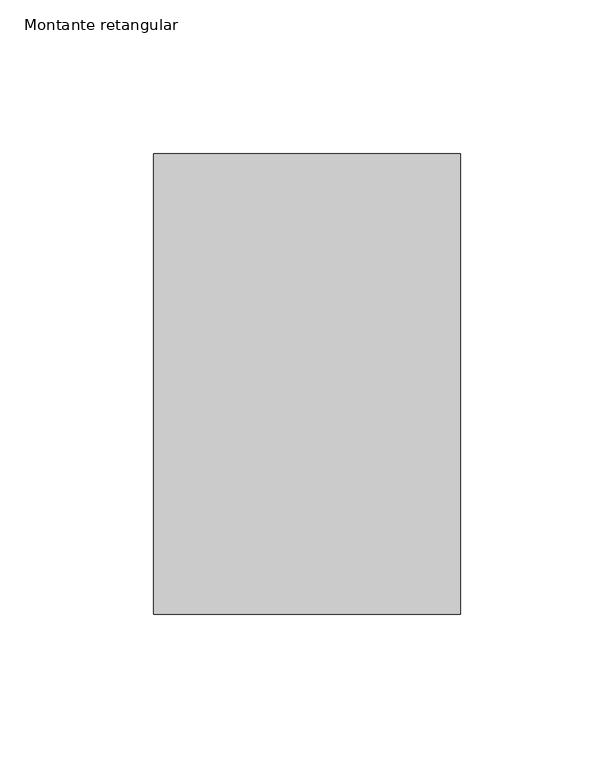
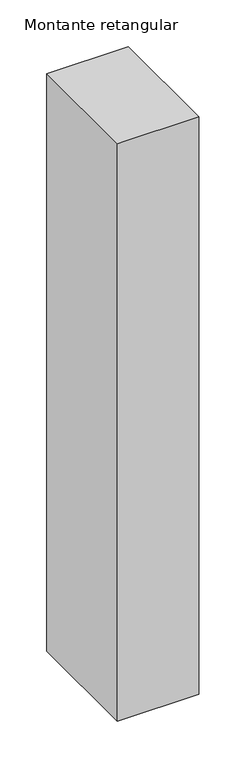
"""IFC4 building model written with IfcOpenShell, lengths in millimetres: member geometry, Montante retangular : CC_100 X 150  mm."""

import ifcopenshell
import ifcopenshell.guid

model = None  # the IFC model being written
_history = None  # IfcOwnerHistory: only IFC2X3 demands one
_inside = {}  # id of a spatial element -> (the spatial element, [elements in it])
_under = {}  # id of a project, library or spatial element -> (it, [spatial elements below it])
_declared = {}  # id of a project -> (the project, [libraries it declares])
_typed = {}  # id of a type object -> (the type object, [elements of that type])
_made_of = {}  # id of a material, layer set ... -> (it, [elements and type objects made of it])


def new_model(schema):
    """Start an empty IFC model of exactly this schema.

    Asked for "IFC4X3", IfcOpenShell would pick the latest addendum, in which some entities
    have other attributes; the version numbers below select the first issue.
    IFC2X3 requires an IfcOwnerHistory on every rooted entity: one is made here for all.
    """
    global model, _history
    if schema == "IFC4X3":
        model = ifcopenshell.file(schema_version=(4, 3, 0, 0))
    else:
        model = ifcopenshell.file(schema=schema)
    _inside.clear()
    _under.clear()
    _declared.clear()
    _typed.clear()
    _made_of.clear()
    _history = None
    if model.schema == "IFC2X3":
        org = make("IfcOrganization", Name="unknown")
        user = make(
            "IfcPersonAndOrganization",
            ThePerson=make("IfcPerson", FamilyName="unknown"),
            TheOrganization=org,
        )
        app = make(
            "IfcApplication",
            ApplicationDeveloper=org,
            Version="unknown",
            ApplicationFullName="unknown",
            ApplicationIdentifier="unknown",
        )
        _history = make(
            "IfcOwnerHistory",
            OwningUser=user,
            OwningApplication=app,
            ChangeAction="ADDED",
            CreationDate=0,
        )
    return model


def make(cls, **values):
    """One entity of the class cls with the attributes given. An attribute that is None is left unset."""
    return model.create_entity(
        cls, **{name: value for name, value in values.items() if value is not None}
    )


def rooted(cls, **values):
    """An entity with a GlobalId (a new one), such as an element, a storey or a relation."""
    return make(cls, GlobalId=ifcopenshell.guid.new(), OwnerHistory=_history, **values)


def si_unit(unit_type, name, prefix=None):
    """IfcSIUnit, for example si_unit("LENGTHUNIT", "METRE", prefix="MILLI")."""
    return make("IfcSIUnit", UnitType=unit_type, Prefix=prefix, Name=name)


def assignment(units):
    """IfcUnitAssignment: the units of a project."""
    return None if units is None else make("IfcUnitAssignment", Units=units)


def point(xyz):
    """IfcCartesianPoint."""
    return None if xyz is None else make("IfcCartesianPoint", Coordinates=xyz)


def direction(xyz):
    """IfcDirection."""
    return None if xyz is None else make("IfcDirection", DirectionRatios=xyz)


def frame(location, z_axis=None, x_axis=None):
    """IfcAxis2Placement3D, a coordinate frame: its origin and axes. An axis left out is left unset."""
    return make(
        "IfcAxis2Placement3D",
        Location=point(location),
        Axis=direction(z_axis),
        RefDirection=direction(x_axis),
    )


def origin():
    """The frame at (0, 0, 0) with its axes left unset."""
    return frame((0.0, 0.0, 0.0))


def place(relative_to, where):
    """IfcLocalPlacement: puts the frame where relative to a parent placement (None: the world)."""
    return make(
        "IfcLocalPlacement", PlacementRelTo=relative_to, RelativePlacement=where
    )


def context(
    kind, dimensions, precision=None, world=None, true_north=None, identifier=None
):
    """IfcGeometricRepresentationContext, for example the 3D "Model" context."""
    return make(
        "IfcGeometricRepresentationContext",
        ContextIdentifier=identifier,
        ContextType=kind,
        CoordinateSpaceDimension=dimensions,
        Precision=precision,
        WorldCoordinateSystem=world,
        TrueNorth=true_north,
    )


def project(units=None, contexts=None):
    """IfcProject with its units and contexts."""
    return rooted(
        "IfcProject",
        Name="project",
        RepresentationContexts=contexts,
        UnitsInContext=assignment(units),
    )


def spatial(cls, under=None, at=None, **own):
    """A site, building, storey or space (cls), placed at a placement, below another one or the project."""
    s = rooted(cls, ObjectPlacement=at, **own)
    if under is not None:
        _under.setdefault(under.id(), (under, []))[1].append(s)
    return s


def polyline(points):
    """IfcPolyline through the points."""
    return make("IfcPolyline", Points=[point(p) for p in points])


def outline(outer, holes=None, kind="AREA"):
    """IfcArbitraryClosedProfileDef: a profile drawn as a closed curve; with holes, ...WithVoids."""
    if holes is None:
        return make("IfcArbitraryClosedProfileDef", ProfileType=kind, OuterCurve=outer)
    return make(
        "IfcArbitraryProfileDefWithVoids",
        ProfileType=kind,
        OuterCurve=outer,
        InnerCurves=holes,
    )


def extrude(swept, where, along, depth):
    """IfcExtrudedAreaSolid: the profile swept, set in the frame where, extruded along a direction by depth."""
    return make(
        "IfcExtrudedAreaSolid",
        SweptArea=swept,
        Position=where,
        ExtrudedDirection=direction(along),
        Depth=depth,
    )


def shape(context_of_items, identifier, shape_type, items):
    """IfcShapeRepresentation: the items that make up one representation, for example the "Body"."""
    return make(
        "IfcShapeRepresentation",
        ContextOfItems=context_of_items,
        RepresentationIdentifier=identifier,
        RepresentationType=shape_type,
        Items=items,
    )


def source(mapping_origin, context_of_items, identifier, shape_type, items):
    """IfcRepresentationMap: a shape defined once, which mapped items show again and again."""
    return make(
        "IfcRepresentationMap",
        MappingOrigin=mapping_origin,
        MappedRepresentation=shape(context_of_items, identifier, shape_type, items),
    )


def transform(
    local_origin,
    x_axis=None,
    y_axis=None,
    z_axis=None,
    scale=None,
    scale2=None,
    scale3=None,
    uniform=True,
):
    """IfcCartesianTransformationOperator3D, or its non-uniform kind. x_axis, y_axis, z_axis: its Axis1, 2, 3."""
    if uniform:
        return make(
            "IfcCartesianTransformationOperator3D",
            Axis1=direction(x_axis),
            Axis2=direction(y_axis),
            LocalOrigin=point(local_origin),
            Scale=scale,
            Axis3=direction(z_axis),
        )
    return make(
        "IfcCartesianTransformationOperator3DnonUniform",
        Axis1=direction(x_axis),
        Axis2=direction(y_axis),
        LocalOrigin=point(local_origin),
        Scale=scale,
        Axis3=direction(z_axis),
        Scale2=scale2,
        Scale3=scale3,
    )


def mapped(mapping_source, mapping_target):
    """IfcMappedItem: shows the shape of a source again, moved by a transform."""
    return make(
        "IfcMappedItem", MappingSource=mapping_source, MappingTarget=mapping_target
    )


def made_of(thing, what):
    """Note that an element or type object is made of a material, layer set ...; save() writes the relation."""
    if what is not None:
        _made_of.setdefault(what.id(), (what, []))[1].append(thing)
    return thing


def element(
    cls,
    number,
    at=None,
    inside=None,
    cuts=None,
    type_object=None,
    material=None,
    context=None,
    identifier="Body",
    shape_type=None,
    held_by="IfcProductDefinitionShape",
    body=None,
    shapes=None,
    **own,
):
    """One element of the class cls, such as IfcWall. Its Tag is "e" and its number.

    at: its placement. inside: the storey or other place that contains it. cuts: it is an
    opening in that element (IfcRelVoidsElement). A single representation is given by context,
    identifier, shape_type and body (its items); several are given by shapes. held_by: the class
    of the entity that holds the representations. save() writes the other relations.
    """
    e = rooted(cls, Tag="e%d" % number, ObjectPlacement=at, **own)
    if body is not None:
        shapes = [shape(context, identifier, shape_type, body)]
    if shapes is not None:
        e.Representation = make(held_by, Representations=shapes)
    if inside is not None:
        _inside.setdefault(inside.id(), (inside, []))[1].append(e)
    if cuts is not None:
        rooted(
            "IfcRelVoidsElement", RelatingBuildingElement=cuts, RelatedOpeningElement=e
        )
    if type_object is not None:
        _typed.setdefault(type_object.id(), (type_object, []))[1].append(e)
    return made_of(e, material)


def aggregate(whole, parts):
    """IfcRelAggregates: a whole, such as a stair, and the parts it consists of."""
    return rooted("IfcRelAggregates", RelatingObject=whole, RelatedObjects=parts)


def save(model, path):
    """Write the relations noted so far, then the file.

    IfcRelAggregates (storeys below a building ...), IfcRelContainedInSpatialStructure (elements
    in a storey), IfcRelDefinesByType, IfcRelAssociatesMaterial and IfcRelDeclares: one each for
    every whole, place, type object, material and project.
    """
    for whole, parts in _under.values():
        aggregate(whole, parts)
    for where, things in _inside.values():
        rooted(
            "IfcRelContainedInSpatialStructure",
            RelatedElements=things,
            RelatingStructure=where,
        )
    for kind, things in _typed.values():
        rooted("IfcRelDefinesByType", RelatedObjects=things, RelatingType=kind)
    for what, things in _made_of.values():
        rooted("IfcRelAssociatesMaterial", RelatedObjects=things, RelatingMaterial=what)
    for by, libraries in _declared.values():
        rooted("IfcRelDeclares", RelatingContext=by, RelatedDefinitions=libraries)
    model.write(path)


def montante_retangular_ab766952(model_context):
    return source(origin(), model_context, "Body", "SweptSolid", [
        extrude(outline(polyline([(50.0, 75.0), (50.0, -75.0), (-50.0, -75.0), (-50.0, 75.0), (50.0, 75.0)])), frame((0.0, 0.0, -750.0), z_axis=(0.0, 0.0, 1.0), x_axis=(1.0, 0.0, 0.0)), (0.0, 0.0, 1.0), 750.0),
    ])


if __name__ == "__main__":
    model = new_model("IFC4")
    model_context = context("Model", 3, world=origin())
    ifc_project = project(units=[si_unit("LENGTHUNIT", "METRE", prefix="MILLI")], contexts=[model_context])
    site = spatial("IfcSite", under=ifc_project)
    building = spatial("IfcBuilding", under=site)
    placement = place(None, origin())
    montante_retangular_shape = montante_retangular_ab766952(model_context)
    element("IfcMember", 1, ObjectType="Montante retangular : CC_100 X 150  mm", at=placement, inside=building, context=model_context, shape_type="MappedRepresentation", body=[
        mapped(montante_retangular_shape, transform((0.0, 0.0, 0.0), x_axis=(1.0, 0.0, 0.0), y_axis=(0.0, 1.0, 0.0), z_axis=(0.0, 0.0, 1.0))),
    ])
    save(model, "model.ifc")

# Revit data of these elements
# Type "Montante retangular : CC_100 X 150  mm"
#   built-in parameter 1007304 = 0.492126 (stored number, unit not read)
#   built-in parameter 1007301 = 0.164042 (stored number, unit not read)
#   built-in parameter 1007300 = 0.164042 (stored number, unit not read)
# Element 1 (IfcMember, "Montante retangular : CC_100 X 150  mm")
#   Materials on its faces: ".ALUMÍNIO"
# Materials
#   ".ALUMÍNIO": class "CC_METAIS", colour RGB 244 244 244, transparency 0, Description = "Material alumínio", Cost = 0
